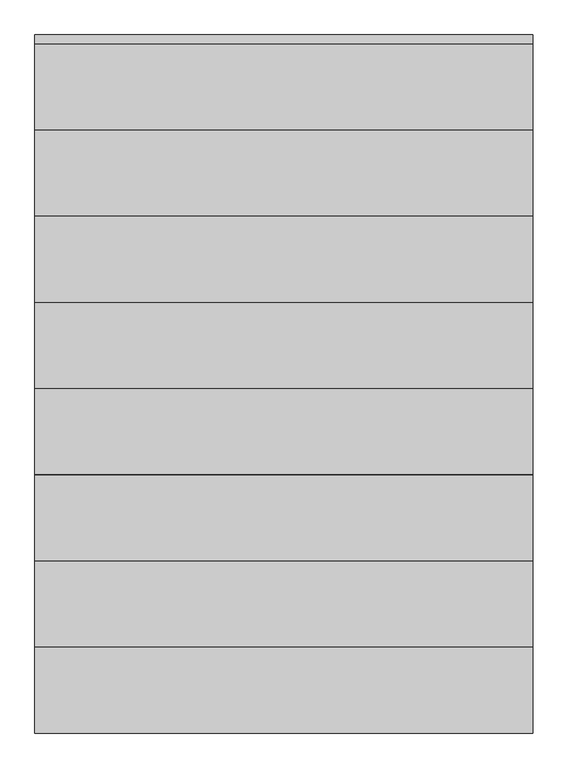
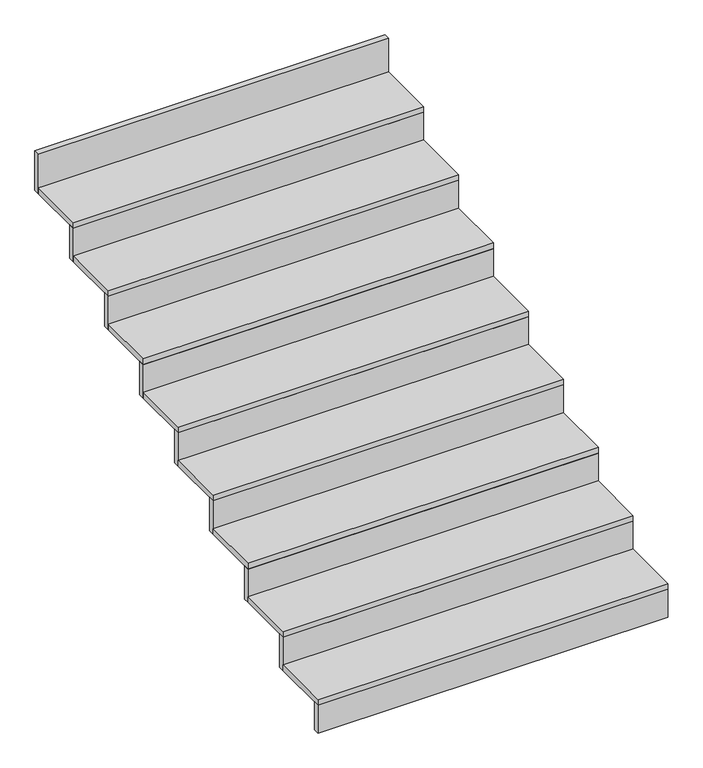
"""IFC4 building model written with IfcOpenShell, lengths in millimetres: stair flight geometry."""

from ifc_helpers import new_model, si_unit, frame, origin, place, context, project, spatial, polyline, outline, extrude, source, transform, mapped, element, save


def stair_flight_14faf888(model_context):
    return source(origin(), model_context, "Body", "SweptSolid", [
        extrude(outline(polyline([(52810.0, -5020.0), (52810.0, -5050.0), (51075.0, -5050.0), (51075.0, -5020.0), (52810.0, -5020.0)])), frame((0.0, 0.0, 10600.0), z_axis=(0.0, 0.0, 1.0), x_axis=(1.0, 0.0, 0.0)), (0.0, 0.0, 1.0), 145.0),
        extrude(outline(polyline([(51075.0, -4750.0), (52810.0, -4750.0), (52810.0, -5050.0), (51075.0, -5050.0), (51075.0, -4750.0)])), frame((0.0, 0.0, 10745.0), z_axis=(0.0, 0.0, 1.0), x_axis=(1.0, 0.0, 0.0)), (0.0, 0.0, 1.0), 30.0),
        extrude(outline(polyline([(52810.0, -4720.0), (52810.0, -4750.0), (51075.0, -4750.0), (51075.0, -4720.0), (52810.0, -4720.0)])), frame((0.0, 0.0, 10745.0), z_axis=(0.0, 0.0, 1.0), x_axis=(1.0, 0.0, 0.0)), (0.0, 0.0, 1.0), 175.0),
        extrude(outline(polyline([(51075.0, -4450.0), (52810.0, -4450.0), (52810.0, -4750.0), (51075.0, -4750.0), (51075.0, -4450.0)])), frame((0.0, 0.0, 10920.0), z_axis=(0.0, 0.0, 1.0), x_axis=(1.0, 0.0, 0.0)), (0.0, 0.0, 1.0), 30.0),
        extrude(outline(polyline([(52810.0, -4420.0), (52810.0, -4450.0), (51075.0, -4450.0), (51075.0, -4420.0), (52810.0, -4420.0)])), frame((0.0, 0.0, 10920.0), z_axis=(0.0, 0.0, 1.0), x_axis=(1.0, 0.0, 0.0)), (0.0, 0.0, 1.0), 175.0),
        extrude(outline(polyline([(51075.0, -4150.0), (52810.0, -4150.0), (52810.0, -4450.0), (51075.0, -4450.0), (51075.0, -4150.0)])), frame((0.0, 0.0, 11095.0), z_axis=(0.0, 0.0, 1.0), x_axis=(1.0, 0.0, 0.0)), (0.0, 0.0, 1.0), 30.0),
        extrude(outline(polyline([(52810.0, -4120.0), (52810.0, -4150.0), (51075.0, -4150.0), (51075.0, -4120.0), (52810.0, -4120.0)])), frame((0.0, 0.0, 11095.0), z_axis=(0.0, 0.0, 1.0), x_axis=(1.0, 0.0, 0.0)), (0.0, 0.0, 1.0), 175.0),
        extrude(outline(polyline([(51075.0, -3850.0), (52810.0, -3850.0), (52810.0, -4150.0), (51075.0, -4150.0), (51075.0, -3850.0)])), frame((0.0, 0.0, 11270.0), z_axis=(0.0, 0.0, 1.0), x_axis=(1.0, 0.0, 0.0)), (0.0, 0.0, 1.0), 30.0),
        extrude(outline(polyline([(52810.0, -3820.0), (52810.0, -3850.0), (51075.0, -3850.0), (51075.0, -3820.0), (52810.0, -3820.0)])), frame((0.0, 0.0, 11270.0), z_axis=(0.0, 0.0, 1.0), x_axis=(1.0, 0.0, 0.0)), (0.0, 0.0, 1.0), 175.0),
        extrude(outline(polyline([(51075.0, -3550.0), (52810.0, -3550.0), (52810.0, -3850.0), (51075.0, -3850.0), (51075.0, -3550.0)])), frame((0.0, 0.0, 11445.0), z_axis=(0.0, 0.0, 1.0), x_axis=(1.0, 0.0, 0.0)), (0.0, 0.0, 1.0), 30.0),
        extrude(outline(polyline([(52810.0, -3520.0), (52810.0, -3550.0), (51075.0, -3550.0), (51075.0, -3520.0), (52810.0, -3520.0)])), frame((0.0, 0.0, 11445.0), z_axis=(0.0, 0.0, 1.0), x_axis=(1.0, 0.0, 0.0)), (0.0, 0.0, 1.0), 175.0),
        extrude(outline(polyline([(51075.0, -3250.0), (52810.0, -3250.0), (52810.0, -3550.0), (51075.0, -3550.0), (51075.0, -3250.0)])), frame((0.0, 0.0, 11620.0), z_axis=(0.0, 0.0, 1.0), x_axis=(1.0, 0.0, 0.0)), (0.0, 0.0, 1.0), 30.0),
        extrude(outline(polyline([(52810.0, -3220.0), (52810.0, -3250.0), (51075.0, -3250.0), (51075.0, -3220.0), (52810.0, -3220.0)])), frame((0.0, 0.0, 11620.0), z_axis=(0.0, 0.0, 1.0), x_axis=(1.0, 0.0, 0.0)), (0.0, 0.0, 1.0), 175.0),
        extrude(outline(polyline([(51075.0, -2950.0), (52810.0, -2950.0), (52810.0, -3250.0), (51075.0, -3250.0), (51075.0, -2950.0)])), frame((0.0, 0.0, 11795.0), z_axis=(0.0, 0.0, 1.0), x_axis=(1.0, 0.0, 0.0)), (0.0, 0.0, 1.0), 30.0),
        extrude(outline(polyline([(52810.0, -2920.0), (52810.0, -2950.0), (51075.0, -2950.0), (51075.0, -2920.0), (52810.0, -2920.0)])), frame((0.0, 0.0, 11795.0), z_axis=(0.0, 0.0, 1.0), x_axis=(1.0, 0.0, 0.0)), (0.0, 0.0, 1.0), 175.0),
        extrude(outline(polyline([(52810.0, -2620.0), (52810.0, -2650.0), (51075.0, -2650.0), (51075.0, -2620.0), (52810.0, -2620.0)])), frame((0.0, 0.0, 11970.0), z_axis=(0.0, 0.0, 1.0), x_axis=(1.0, 0.0, 0.0)), (0.0, 0.0, 1.0), 205.0),
        extrude(outline(polyline([(51075.0, -2650.0), (52810.0, -2650.0), (52810.0, -2950.0), (51075.0, -2950.0), (51075.0, -2650.0)])), frame((0.0, 0.0, 11970.0), z_axis=(0.0, 0.0, 1.0), x_axis=(1.0, 0.0, 0.0)), (0.0, 0.0, 1.0), 30.0),
    ])


if __name__ == "__main__":
    model = new_model("IFC4")
    model_context = context("Model", 3, world=origin())
    ifc_project = project(units=[si_unit("LENGTHUNIT", "METRE", prefix="MILLI")], contexts=[model_context])
    site = spatial("IfcSite", under=ifc_project)
    building = spatial("IfcBuilding", under=site)
    placement = place(None, origin())
    stair_flight_shape = stair_flight_14faf888(model_context)
    element("IfcStairFlight", 1, at=placement, inside=building, context=model_context, shape_type="MappedRepresentation", body=[
        mapped(stair_flight_shape, transform((0.0, 0.0, 0.0), x_axis=(1.0, 0.0, 0.0), y_axis=(0.0, 1.0, 0.0), z_axis=(0.0, 0.0, 1.0))),
    ])
    save(model, "model.ifc")

# Revit data of these elements
# Element 1 (IfcStairFlight)
#   Materials on its faces: "00_Finish_Deco Tile"
# Materials
#   "00_Finish_Deco Tile": class "Finish", colour RGB 245 245 245, transparency 0, Description = "Ceramic Tile", Cost = 0
